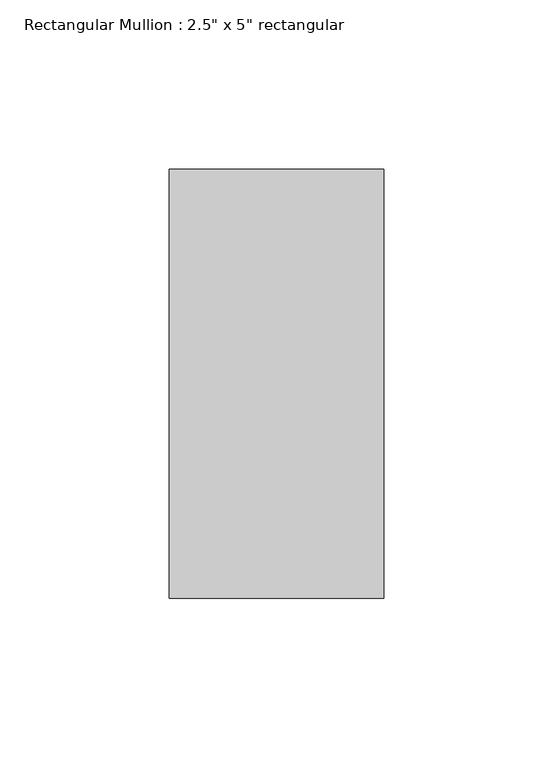
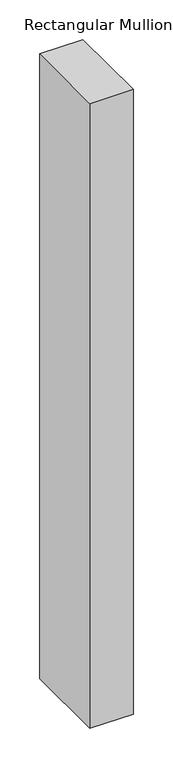
"""IFC4 building model written with IfcOpenShell, lengths in millimetres: member geometry."""

from ifc_helpers import new_model, si_unit, frame, origin, place, context, project, spatial, polyline, outline, extrude, source, transform, mapped, element, save


def member_1f3bd77c(model_context):
    return source(origin(), model_context, "Body", "SweptSolid", [
        extrude(outline(polyline([(0.0, 63.5), (0.0, -63.5), (-63.5, -63.5), (-63.5, 63.5), (0.0, 63.5)])), frame((0.0, 0.0, -965.1999998), z_axis=(0.0, 0.0, 1.0), x_axis=(1.0, 0.0, 0.0)), (0.0, 0.0, 1.0), 965.1999998),
    ])


if __name__ == "__main__":
    model = new_model("IFC4")
    model_context = context("Model", 3, world=origin())
    ifc_project = project(units=[si_unit("LENGTHUNIT", "METRE", prefix="MILLI")], contexts=[model_context])
    site = spatial("IfcSite", under=ifc_project)
    building = spatial("IfcBuilding", under=site)
    placement = place(None, origin())
    member_shape = member_1f3bd77c(model_context)
    element("IfcMember", 1, ObjectType="Rectangular Mullion : 2.5\" x 5\" rectangular", at=placement, inside=building, context=model_context, shape_type="MappedRepresentation", body=[
        mapped(member_shape, transform((0.0, 0.0, 0.0), x_axis=(1.0, 0.0, 0.0), y_axis=(0.0, 1.0, 0.0), z_axis=(0.0, 0.0, 1.0))),
    ])
    save(model, "model.ifc")

# Revit data of these elements
# Type "Rectangular Mullion : 2.5\" x 5\" rectangular"
#   built-in parameter 1007304 = 0.416667 (stored number, unit not read)
#   built-in parameter 1007301 = 0.104167 (stored number, unit not read)
#   built-in parameter 1007300 = 0.104167 (stored number, unit not read)
# Element 1 (IfcMember, "Rectangular Mullion : 2.5\" x 5\" rectangular")
#   Materials on its faces: "Aluminum"
# Materials
#   "Aluminum": class "Metal", colour RGB 247 247 247, transparency 0, Description = "Aluminum 6061", Cost = 0
